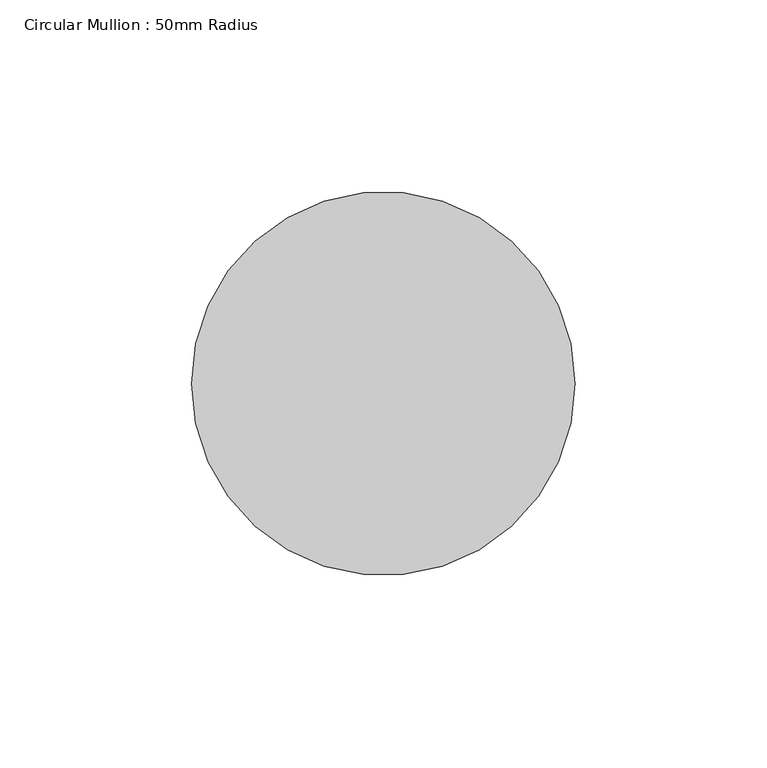
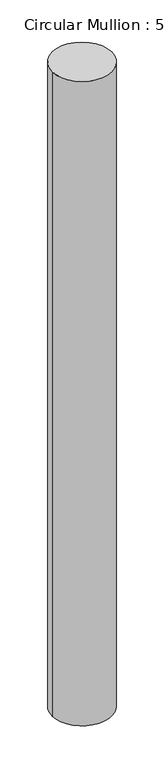
"""IFC4 building model written with IfcOpenShell, lengths in millimetres: member geometry, Circular Mullion : 50mm Radius."""

from ifc_helpers import new_model, si_unit, point, frame, origin, origin_2d, place, context, project, spatial, circle_curve, trimmed, segment, composite_curve, outline, extrude, source, transform, mapped, element, save


def circular_mullion_50mm_radius_29e0157e(model_context):
    return source(origin(), model_context, "Body", "SweptSolid", [
        extrude(outline(composite_curve([segment(trimmed(circle_curve(origin_2d(), 50.0), [point((50.0, 0.0))], [point((-50.0, 0.0))], False, "CARTESIAN"), True, "CONTINUOUS"), segment(trimmed(circle_curve(origin_2d(), 50.0), [point((-50.0, 0.0))], [point((50.0, 0.0))], False, "CARTESIAN"), True, "CONTINUOUS")], self_intersect=False)), frame((0.0, 0.0, -1144.047787), z_axis=(0.0, 0.0, 1.0), x_axis=(1.0, 0.0, 0.0)), (0.0, 0.0, 1.0), 1144.047787),
    ])


if __name__ == "__main__":
    model = new_model("IFC4")
    model_context = context("Model", 3, world=origin())
    ifc_project = project(units=[si_unit("LENGTHUNIT", "METRE", prefix="MILLI")], contexts=[model_context])
    site = spatial("IfcSite", under=ifc_project)
    building = spatial("IfcBuilding", under=site)
    placement = place(None, origin())
    circular_mullion_50mm_radius_shape = circular_mullion_50mm_radius_29e0157e(model_context)
    element("IfcMember", 1, ObjectType="Circular Mullion : 50mm Radius", at=placement, inside=building, context=model_context, shape_type="MappedRepresentation", body=[
        mapped(circular_mullion_50mm_radius_shape, transform((0.0, 0.0, 0.0), x_axis=(1.0, 0.0, 0.0), y_axis=(0.0, 1.0, 0.0), z_axis=(0.0, 0.0, 1.0))),
    ])
    save(model, "model.ifc")

# Revit data of these elements
# Type "Circular Mullion : 50mm Radius"
#   built-in parameter 1007350 = 0.164042 (stored number, unit not read)
# Element 1 (IfcMember, "Circular Mullion : 50mm Radius")
#   Materials on its faces: "Aluminium"
# Materials
#   "Aluminium": class "Metal", colour RGB 247 247 247, transparency 0, Description = "Aluminium 6061", Cost = 0
